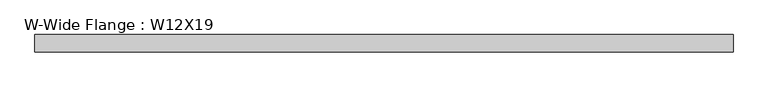
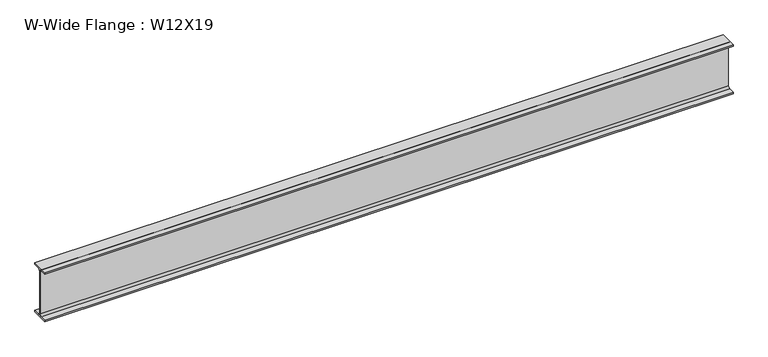
"""IFC4 building model written with IfcOpenShell, lengths in millimetres: beam geometry, W-Wide Flange : W12X19."""

from ifc_helpers import new_model, si_unit, point, frame, frame_2d, origin, place, context, project, spatial, polyline, circle_curve, trimmed, segment, composite_curve, outline, extrude, source, transform, mapped, element, save


def w_wide_flange_w12x19_3c6426ae(model_context):
    return source(origin(), model_context, "Body", "SweptSolid", [
        extrude(outline(composite_curve([segment(polyline([(50.927, -146.05), (50.927, -154.94), (-50.927, -154.94), (-50.927, -146.05), (-16.3195, -146.05)]), True, "CONTINUOUS"), segment(trimmed(circle_curve(frame_2d((-16.3195, -132.715)), 13.335), [point((-16.3195, -146.05))], [point((-2.9845, -132.715))], True, "CARTESIAN"), True, "CONTINUOUS"), segment(polyline([(-2.9845, -132.715), (-2.9845, 132.715)]), True, "CONTINUOUS"), segment(trimmed(circle_curve(frame_2d((-16.3195, 132.715)), 13.335), [point((-2.9845, 132.715))], [point((-16.3195, 146.05))], True, "CARTESIAN"), True, "CONTINUOUS"), segment(polyline([(-16.3195, 146.05), (-50.927, 146.05), (-50.927, 154.94), (50.927, 154.94), (50.927, 146.05), (16.3195, 146.05)]), True, "CONTINUOUS"), segment(trimmed(circle_curve(frame_2d((16.3195, 132.715)), 13.335), [point((16.3195, 146.05))], [point((2.9845, 132.715))], True, "CARTESIAN"), True, "CONTINUOUS"), segment(polyline([(2.9845, 132.715), (2.9845, -132.715)]), True, "CONTINUOUS"), segment(trimmed(circle_curve(frame_2d((16.3195, -132.715)), 13.335), [point((2.9845, -132.715))], [point((16.3195, -146.05))], True, "CARTESIAN"), True, "CONTINUOUS"), segment(polyline([(16.3195, -146.05), (50.927, -146.05)]), True, "CONTINUOUS")], self_intersect=False)), frame((-2032.0, 0.0, 0.0), z_axis=(1.0, 0.0, 0.0), x_axis=(0.0, 1.0, 0.0)), (0.0, 0.0, 1.0), 4114.8),
    ])


if __name__ == "__main__":
    model = new_model("IFC4")
    model_context = context("Model", 3, world=origin())
    ifc_project = project(units=[si_unit("LENGTHUNIT", "METRE", prefix="MILLI")], contexts=[model_context])
    site = spatial("IfcSite", under=ifc_project)
    building = spatial("IfcBuilding", under=site)
    placement = place(None, origin())
    w_wide_flange_w12x19_shape = w_wide_flange_w12x19_3c6426ae(model_context)
    element("IfcBeam", 1, ObjectType="W-Wide Flange : W12X19", at=placement, inside=building, context=model_context, shape_type="MappedRepresentation", body=[
        mapped(w_wide_flange_w12x19_shape, transform((0.0, 0.0, 0.0), x_axis=(1.0, 0.0, 0.0), y_axis=(0.0, 1.0, 0.0), z_axis=(0.0, 0.0, 1.0))),
    ])
    save(model, "model.ifc")

# Revit data of these elements
# Type "W-Wide Flange : W12X19"
#   Assembly Code = "B10"
#   W = 19
#   Length [instance default] = 5' - 0"
#   bf = 0' - 4.01"
#   d = 1' - 0.2"
#   k = 0' - 0 7/8"
#   k2 = 0' - 0.525"
#   tf = 0' - 0.35"
#   tw = 0' - 0.235"
#   A = 0.0386806 SF
#   Structural Material [instance default] = Steel ASTM A992
# Element 1 (IfcBeam, "W-Wide Flange : W12X19")
#   Materials on its faces: "Steel ASTM A992"
# Materials
#   "Steel ASTM A992": class "Metal", colour RGB 199 199 199, transparency 0, Description = "Structural steel 50ksi", Cost = 0
